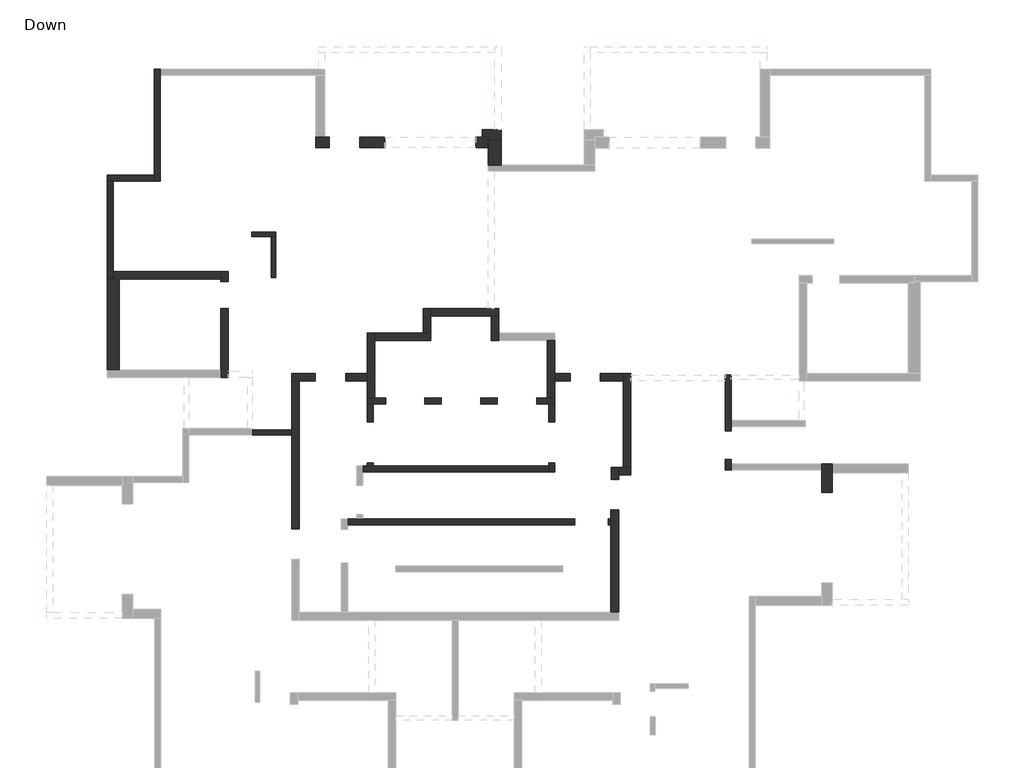
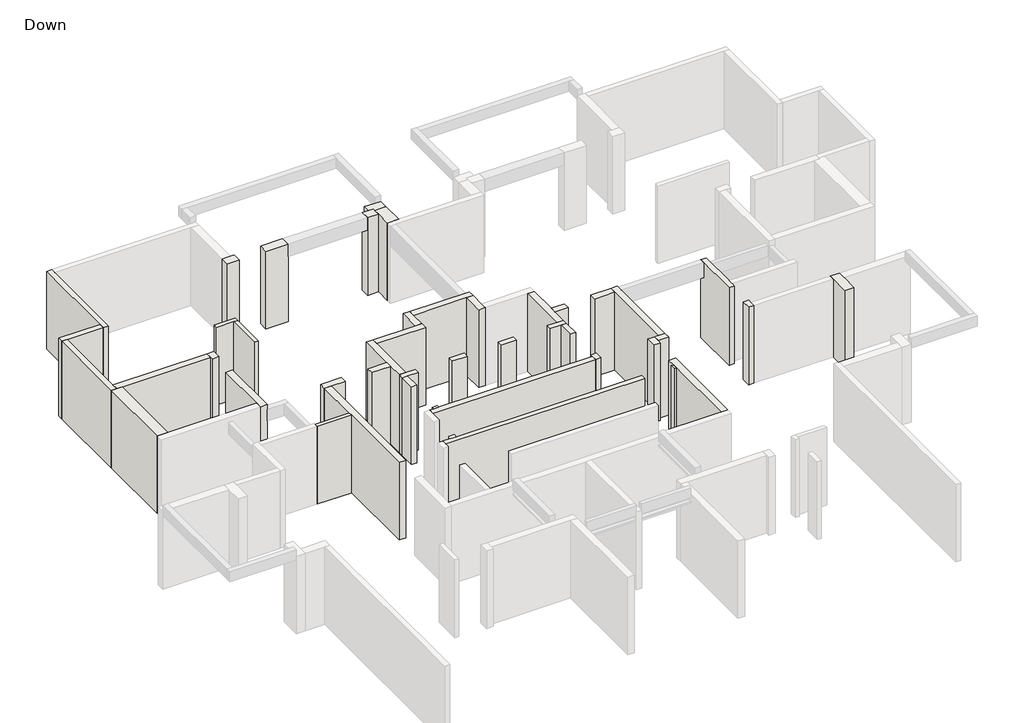
# One storey, part 2 of 3: 44 walls.
"""IFC4 building model written with IfcOpenShell, lengths in millimetres."""

from ifc_helpers import new_model, si_unit, origin, place, context, project, spatial, faceted_brep, element, save

model = new_model("IFC4")

# Units and contexts
model_context = context("Model", 3, world=origin())
ifc_project = project(units=[si_unit("LENGTHUNIT", "METRE", prefix="MILLI")], contexts=[model_context])

# Site, building, storey
site = spatial("IfcSite", under=ifc_project)
building = spatial("IfcBuilding", under=site)
storey = spatial("IfcBuildingStorey", under=building, Name="Down", Elevation=0.0)

# Walls
placement = place(None, origin())
element("IfcWall", 1, ObjectType="15", at=placement, inside=storey, context=model_context, shape_type="Brep", body=[
    faceted_brep([(7954.0579731, -10774.5447275, 0.0), (9252.6267863, -10774.5447275, 0.0), (9252.6267863, -10774.5447275, 2730.0), (9252.6267863, -10774.5447275, 2950.0), (9252.6267863, -10774.5447275, 3100.0), (7954.0579731, -10774.5447275, 3100.0), (7954.0579731, -10624.5447275, 0.0), (7954.0579731, -10624.5447275, 3100.0), (9252.6267863, -10624.5447275, 3100.0), (9252.6267863, -10624.5447275, 0.0)], [[[0, 1, 2, 3, 4, 5]], [[6, 7, 8, 9]], [[1, 0, 6, 9]], [[5, 4, 8, 7]], [[0, 5, 7, 6]], [[4, 3, 2, 1, 9, 8]]]),
])
element("IfcWall", 2, ObjectType="15", at=placement, inside=storey, context=model_context, shape_type="Brep", body=[
    faceted_brep([(7932.894282, -4226.5861029, 0.0), (8577.767247, -4226.5861029, 0.0), (8727.767247, -4226.5861029, 0.0), (8727.767247, -4226.5861029, 3100.0), (8577.767247, -4226.5861029, 3100.0), (7932.894282, -4226.5861029, 3100.0), (7932.894282, -4226.5861029, 2950.0), (7932.894282, -4226.5861029, 2730.0), (7932.894282, -4076.5861029, 0.0), (7932.894282, -4076.5861029, 2730.0), (7932.894282, -4076.5861029, 2950.0), (7932.894282, -4076.5861029, 3100.0), (8727.767247, -4076.5861029, 3100.0), (8727.767247, -4076.5861029, 2950.0), (8727.767247, -4076.5861029, 2730.0), (8727.767247, -4076.5861029, 0.0)], [[[0, 1, 2, 3, 4, 5, 6, 7]], [[8, 9, 10, 11, 12, 13, 14, 15]], [[2, 1, 0, 8, 15]], [[5, 4, 3, 12, 11]], [[0, 7, 6, 5, 11, 10, 9, 8]], [[3, 2, 15, 14, 13, 12]]]),
])
element("IfcWall", 3, ObjectType="15", at=placement, inside=storey, context=model_context, shape_type="Brep", body=[
    faceted_brep([(8577.767247, -4226.5861029, 0.0), (8577.767247, -5575.151797, 0.0), (8577.767247, -5575.151797, 2730.0), (8577.767247, -5575.151797, 2950.0), (8577.767247, -5575.151797, 3100.0), (8577.767247, -4226.5861029, 3100.0), (8577.767247, -4226.5861029, 2950.0), (8577.767247, -4226.5861029, 2730.0), (8727.767247, -4226.5861029, 0.0), (8727.767247, -4226.5861029, 3100.0), (8727.767247, -5575.151797, 3100.0), (8727.767247, -5575.151797, 2950.0), (8727.767247, -5575.151797, 2730.0), (8727.767247, -5575.151797, 0.0)], [[[0, 1, 2, 3, 4, 5, 6, 7]], [[8, 9, 10, 11, 12, 13]], [[1, 0, 8, 13]], [[4, 3, 2, 1, 13, 12, 11, 10]], [[5, 4, 10, 9]], [[0, 7, 6, 5, 9, 8]]]),
])
element("IfcWall", 4, ObjectType="20", at=placement, inside=storey, context=model_context, shape_type="Brep", body=[
    faceted_brep([(4715.8368705, 1316.275118, 0.0), (4715.8368705, -2183.1380866, 0.0), (4715.8368705, -2383.1380866, 0.0), (4715.8368705, -2383.1380866, 3100.0), (4715.8368705, -2183.1380866, 3100.0), (4715.8368705, 1316.275118, 3100.0), (4915.8368705, 1316.275118, 0.0), (4915.8368705, 1316.275118, 3100.0), (4915.8368705, 1116.275118, 3100.0), (4915.8368705, -2383.1380866, 3100.0), (4915.8368705, -2383.1380866, 2950.0), (4915.8368705, -2383.1380866, 2730.0), (4915.8368705, -2383.1380866, 0.0), (4915.8368705, 1116.275118, 0.0)], [[[0, 1, 2, 3, 4, 5]], [[6, 7, 8, 9, 10, 11, 12, 13]], [[2, 1, 0, 6, 13, 12]], [[5, 4, 3, 9, 8, 7]], [[3, 2, 12, 11, 10, 9]], [[0, 5, 7, 6]]]),
])
element("IfcWall", 5, ObjectType="20", at=placement, inside=storey, context=model_context, shape_type="Brep", body=[
    faceted_brep([(4715.8368705, -2183.1380866, 0.0), (3157.3073849, -2183.1380866, 0.0), (3157.3073849, -2183.1380866, 3100.0), (4715.8368705, -2183.1380866, 3100.0), (4715.8368705, -2383.1380866, 0.0), (4715.8368705, -2383.1380866, 3100.0), (3357.3073849, -2383.1380866, 3100.0), (3157.3073849, -2383.1380866, 3100.0), (3157.3073849, -2383.1380866, 0.0), (3357.3073849, -2383.1380866, 0.0)], [[[0, 1, 2, 3]], [[4, 5, 6, 7, 8, 9]], [[1, 0, 4, 9, 8]], [[3, 2, 7, 6, 5]], [[0, 3, 5, 4]], [[2, 1, 8, 7]]]),
])
element("IfcWall", 6, ObjectType="20", at=placement, inside=storey, context=model_context, shape_type="Brep", body=[
    faceted_brep([(3157.3073849, -2383.1380866, 0.0), (3157.3073849, -5626.3894647, 0.0), (3157.3073849, -5626.3894647, 3100.0), (3157.3073849, -2383.1380866, 3100.0), (3357.3073849, -2383.1380866, 0.0), (3357.3073849, -2383.1380866, 2730.0), (3357.3073849, -2383.1380866, 2950.0), (3357.3073849, -2383.1380866, 3100.0), (3357.3073849, -5376.3894647, 3100.0), (3357.3073849, -5626.3894647, 3100.0), (3357.3073849, -5626.3894647, 0.0), (3357.3073849, -5376.3894647, 0.0)], [[[0, 1, 2, 3]], [[4, 5, 6, 7, 8, 9, 10, 11]], [[1, 0, 4, 11, 10]], [[3, 2, 9, 8, 7]], [[0, 3, 7, 6, 5, 4]], [[2, 1, 10, 9]]]),
])
element("IfcWall", 7, ObjectType="20", at=placement, inside=storey, context=model_context, shape_type="Brep", body=[
    faceted_brep([(23780.6220263, -11933.0804512, 0.0), (23780.6220263, -11733.0804512, 0.0), (23780.6220263, -11585.6400699, 0.0), (23780.6220263, -11585.6400699, 3100.0), (23780.6220263, -11733.0804512, 3100.0), (23780.6220263, -11933.0804512, 3100.0), (23580.6220263, -11933.0804512, 0.0), (23580.6220263, -11933.0804512, 2730.0), (23580.6220263, -11933.0804512, 2950.0), (23580.6220263, -11933.0804512, 3100.0), (23580.6220263, -11585.6400699, 3100.0), (23580.6220263, -11585.6400699, 0.0)], [[[0, 1, 2, 3, 4, 5]], [[6, 7, 8, 9, 10, 11]], [[2, 1, 0, 6, 11]], [[3, 2, 11, 10]], [[5, 4, 3, 10, 9]], [[0, 5, 9, 8, 7, 6]]]),
])
element("IfcWall", 8, ObjectType="20", at=placement, inside=storey, context=model_context, shape_type="Brep", body=[
    faceted_brep([(23780.6220263, -10650.7340155, 0.0), (23780.6220263, -10505.7627314, 0.0), (23780.6220263, -10305.7627314, 0.0), (23780.6220263, -8804.7310591, 0.0), (23780.6220263, -8804.7310591, 2300.0), (23780.6220263, -8804.7310591, 2450.0), (23780.6220263, -8804.7310591, 2900.0), (23780.6220263, -8804.7310591, 3100.0), (23780.6220263, -10305.7627314, 3100.0), (23780.6220263, -10505.7627314, 3100.0), (23780.6220263, -10650.7340155, 3100.0), (23580.6220263, -10650.7340155, 0.0), (23580.6220263, -10650.7340155, 3100.0), (23580.6220263, -8804.7310591, 3100.0), (23580.6220263, -8804.7310591, 0.0)], [[[0, 1, 2, 3, 4, 5, 6, 7, 8, 9, 10]], [[11, 12, 13, 14]], [[3, 2, 1, 0, 11, 14]], [[7, 6, 5, 4, 3, 14, 13]], [[10, 9, 8, 7, 13, 12]], [[0, 10, 12, 11]]]),
])
element("IfcWall", 9, ObjectType="20", at=placement, inside=storey, context=model_context, shape_type="Brep", body=[
    faceted_brep([(17955.1365674, -9553.3935127, 0.0), (17705.1365674, -9553.3935127, 0.0), (17354.0877401, -9553.3935127, 0.0), (17354.0877401, -9553.3935127, 3100.0), (17705.1365674, -9553.3935127, 3100.0), (17955.1365674, -9553.3935127, 3100.0), (17955.1365674, -9753.3935127, 0.0), (17955.1365674, -9753.3935127, 3100.0), (17755.1365674, -9753.3935127, 3100.0), (17354.0877401, -9753.3935127, 3100.0), (17354.0877401, -9753.3935127, 2950.0), (17354.0877401, -9753.3935127, 2730.0), (17354.0877401, -9753.3935127, 0.0), (17755.1365674, -9753.3935127, 0.0)], [[[0, 1, 2, 3, 4, 5]], [[6, 7, 8, 9, 10, 11, 12, 13]], [[2, 1, 0, 6, 13, 12]], [[3, 2, 12, 11, 10, 9]], [[5, 4, 3, 9, 8, 7]], [[0, 5, 7, 6]]]),
])
element("IfcWall", 10, ObjectType="20", at=placement, inside=storey, context=model_context, shape_type="Brep", body=[
    faceted_brep([(16055.5189269, -9553.3966318, 0.0), (15504.3811378, -9553.3966318, 0.0), (15504.3811378, -9553.3966318, 2730.0), (15504.3811378, -9553.3966318, 2950.0), (15504.3811378, -9553.3966318, 3100.0), (16055.5189269, -9553.3966318, 3100.0), (16055.5189269, -9553.3966318, 2950.0), (16055.5189269, -9553.3966318, 2730.0), (16055.5189269, -9753.3966318, 0.0), (16055.5189269, -9753.3966318, 2730.0), (16055.5189269, -9753.3966318, 2950.0), (16055.5189269, -9753.3966318, 3100.0), (15504.3811378, -9753.3966318, 3100.0), (15504.3811378, -9753.3966318, 2950.0), (15504.3811378, -9753.3966318, 2730.0), (15504.3811378, -9753.3966318, 0.0)], [[[0, 1, 2, 3, 4, 5, 6, 7]], [[8, 9, 10, 11, 12, 13, 14, 15]], [[1, 0, 8, 15]], [[4, 3, 2, 1, 15, 14, 13, 12]], [[5, 4, 12, 11]], [[0, 7, 6, 5, 11, 10, 9, 8]]]),
])
element("IfcWall", 11, ObjectType="20", at=placement, inside=storey, context=model_context, shape_type="Brep", body=[
    faceted_brep([(14205.8123246, -9553.3966318, 0.0), (13654.4981714, -9553.3966318, 0.0), (13654.4981714, -9553.3966318, 2730.0), (13654.4981714, -9553.3966318, 2950.0), (13654.4981714, -9553.3966318, 3100.0), (14205.8123246, -9553.3966318, 3100.0), (14205.8123246, -9553.3966318, 2950.0), (14205.8123246, -9553.3966318, 2730.0), (14205.8123246, -9753.3966318, 0.0), (14205.8123246, -9753.3966318, 2730.0), (14205.8123246, -9753.3966318, 2950.0), (14205.8123246, -9753.3966318, 3100.0), (13654.4981714, -9753.3966318, 3100.0), (13654.4981714, -9753.3966318, 2950.0), (13654.4981714, -9753.3966318, 2730.0), (13654.4981714, -9753.3966318, 0.0)], [[[0, 1, 2, 3, 4, 5, 6, 7]], [[8, 9, 10, 11, 12, 13, 14, 15]], [[1, 0, 8, 15]], [[4, 3, 2, 1, 15, 14, 13, 12]], [[5, 4, 12, 11]], [[0, 7, 6, 5, 11, 10, 9, 8]]]),
])
element("IfcWall", 12, ObjectType="20", at=placement, inside=storey, context=model_context, shape_type="Brep", body=[
    faceted_brep([(12355.9293582, -9553.3966318, 0.0), (12004.8805309, -9553.3966318, 0.0), (11754.8805309, -9553.3966318, 0.0), (11754.8805309, -9553.3966318, 3100.0), (12004.8805309, -9553.3966318, 3100.0), (12355.9293582, -9553.3966318, 3100.0), (12355.9293582, -9553.3966318, 2950.0), (12355.9293582, -9553.3966318, 2730.0), (12355.9293582, -9753.3966318, 0.0), (12355.9293582, -9753.3966318, 2730.0), (12355.9293582, -9753.3966318, 2950.0), (12355.9293582, -9753.3966318, 3100.0), (11954.8805309, -9753.3966318, 3100.0), (11754.8805309, -9753.3966318, 3100.0), (11754.8805309, -9753.3966318, 0.0), (11954.8805309, -9753.3966318, 0.0)], [[[0, 1, 2, 3, 4, 5, 6, 7]], [[8, 9, 10, 11, 12, 13, 14, 15]], [[2, 1, 0, 8, 15, 14]], [[5, 4, 3, 13, 12, 11]], [[0, 7, 6, 5, 11, 10, 9, 8]], [[3, 2, 14, 13]]]),
])
element("IfcWall", 13, ObjectType="20", at=placement, inside=storey, context=model_context, shape_type="Brep", body=[
    faceted_brep([(11754.8805309, -9753.3966318, 0.0), (11754.8805309, -10353.2077914, 0.0), (11754.8805309, -10353.2077914, 2730.0), (11754.8805309, -10353.2077914, 2950.0), (11754.8805309, -10353.2077914, 3100.0), (11754.8805309, -9753.3966318, 3100.0), (11954.8805309, -9753.3966318, 0.0), (11954.8805309, -9753.3966318, 2730.0), (11954.8805309, -9753.3966318, 2950.0), (11954.8805309, -9753.3966318, 3100.0), (11954.8805309, -10353.2077914, 3100.0), (11954.8805309, -10353.2077914, 2950.0), (11954.8805309, -10353.2077914, 2730.0), (11954.8805309, -10353.2077914, 0.0)], [[[0, 1, 2, 3, 4, 5]], [[6, 7, 8, 9, 10, 11, 12, 13]], [[1, 0, 6, 13]], [[4, 3, 2, 1, 13, 12, 11, 10]], [[5, 4, 10, 9]], [[0, 5, 9, 8, 7, 6]]]),
])
element("IfcWall", 14, ObjectType="20", at=placement, inside=storey, context=model_context, shape_type="Brep", body=[
    faceted_brep([(11754.8805309, -11704.3331041, 0.0), (11754.8805309, -11804.3284255, 0.0), (11754.8805309, -11804.3284255, 2730.0), (11754.8805309, -11804.3284255, 2950.0), (11754.8805309, -11804.3284255, 3100.0), (11754.8805309, -11704.3331041, 3100.0), (11754.8805309, -11704.3331041, 2950.0), (11754.8805309, -11704.3331041, 2730.0), (11954.8805309, -11704.3331041, 0.0), (11954.8805309, -11704.3331041, 2730.0), (11954.8805309, -11704.3331041, 2950.0), (11954.8805309, -11704.3331041, 3100.0), (11954.8805309, -11804.3284255, 3100.0), (11954.8805309, -11804.3284255, 2950.0), (11954.8805309, -11804.3284255, 2730.0), (11954.8805309, -11804.3284255, 0.0)], [[[0, 1, 2, 3, 4, 5, 6, 7]], [[8, 9, 10, 11, 12, 13, 14, 15]], [[1, 0, 8, 15]], [[5, 4, 12, 11]], [[0, 7, 6, 5, 11, 10, 9, 8]], [[4, 3, 2, 1, 15, 14, 13, 12]]]),
])
element("IfcWall", 15, ObjectType="20", at=placement, inside=storey, context=model_context, shape_type="Brep", body=[
    faceted_brep([(11603.5632586, -12004.3284255, 0.0), (17755.1365674, -12004.3284255, 0.0), (17755.1365674, -12004.3284255, 3100.0), (11603.5632586, -12004.3284255, 3100.0), (11603.5632586, -12004.3284255, 2950.0), (11603.5632586, -12004.3284255, 2730.0), (11603.5632586, -11804.3284255, 0.0), (11603.5632586, -11804.3284255, 3100.0), (11754.8805309, -11804.3284255, 3100.0), (11954.8805309, -11804.3284255, 3100.0), (17755.1365674, -11804.3284255, 3100.0), (17755.1365674, -11804.3284255, 2950.0), (17755.1365674, -11804.3284255, 2730.0), (17755.1365674, -11804.3284255, 0.0), (11954.8805309, -11804.3284255, 0.0), (11754.8805309, -11804.3284255, 0.0)], [[[0, 1, 2, 3, 4, 5]], [[6, 7, 8, 9, 10, 11, 12, 13, 14, 15]], [[1, 0, 6, 15, 14, 13]], [[3, 2, 10, 9, 8, 7]], [[2, 1, 13, 12, 11, 10]], [[0, 5, 4, 3, 7, 6]]]),
])
element("IfcWall", 16, ObjectType="20", at=placement, inside=storey, context=model_context, shape_type="Brep", body=[
    faceted_brep([(17955.1365674, -12004.3284255, 0.0), (17955.1365674, -11704.3331041, 0.0), (17955.1365674, -11704.3331041, 2730.0), (17955.1365674, -11704.3331041, 2950.0), (17955.1365674, -11704.3331041, 3100.0), (17955.1365674, -12004.3284255, 3100.0), (17955.1365674, -12004.3284255, 2950.0), (17955.1365674, -12004.3284255, 2730.0), (17755.1365674, -12004.3284255, 0.0), (17755.1365674, -12004.3284255, 3100.0), (17755.1365674, -11804.3284255, 3100.0), (17755.1365674, -11704.3331041, 3100.0), (17755.1365674, -11704.3331041, 2950.0), (17755.1365674, -11704.3331041, 2730.0), (17755.1365674, -11704.3331041, 0.0), (17755.1365674, -11804.3284255, 0.0)], [[[0, 1, 2, 3, 4, 5, 6, 7]], [[8, 9, 10, 11, 12, 13, 14, 15]], [[1, 0, 8, 15, 14]], [[4, 3, 2, 1, 14, 13, 12, 11]], [[5, 4, 11, 10, 9]], [[0, 7, 6, 5, 9, 8]]]),
])
element("IfcWall", 17, ObjectType="20", at=placement, inside=storey, context=model_context, shape_type="Brep", body=[
    faceted_brep([(17755.1365674, -9753.3935127, 0.0), (17755.1365674, -10353.2077914, 0.0), (17755.1365674, -10353.2077914, 2730.0), (17755.1365674, -10353.2077914, 2950.0), (17755.1365674, -10353.2077914, 3100.0), (17755.1365674, -9753.3935127, 3100.0), (17755.1365674, -9753.3935127, 2950.0), (17755.1365674, -9753.3935127, 2730.0), (17955.1365674, -9753.3935127, 0.0), (17955.1365674, -9753.3935127, 3100.0), (17955.1365674, -10353.2077914, 3100.0), (17955.1365674, -10353.2077914, 2950.0), (17955.1365674, -10353.2077914, 2730.0), (17955.1365674, -10353.2077914, 0.0)], [[[0, 1, 2, 3, 4, 5, 6, 7]], [[8, 9, 10, 11, 12, 13]], [[1, 0, 8, 13]], [[4, 3, 2, 1, 13, 12, 11, 10]], [[5, 4, 10, 9]], [[0, 7, 6, 5, 9, 8]]]),
])
element("IfcWall", 18, ObjectType="20", at=placement, inside=storey, context=model_context, shape_type="Brep", body=[
    faceted_brep([(11100.0437745, -13752.8020387, 0.0), (18611.3873556, -13752.8020387, 0.0), (18611.3873556, -13752.8020387, 2730.0), (18611.3873556, -13752.8020387, 2950.0), (18611.3873556, -13752.8020387, 3100.0), (11100.0437745, -13752.8020387, 3100.0), (11100.0437745, -13752.8020387, 2950.0), (11100.0437745, -13752.8020387, 2730.0), (11100.0437745, -13552.8020387, 0.0), (11100.0437745, -13552.8020387, 3100.0), (11403.5632586, -13552.8020387, 3100.0), (11603.5632586, -13552.8020387, 3100.0), (18611.3873556, -13552.8020387, 3100.0), (18611.3873556, -13552.8020387, 2950.0), (18611.3873556, -13552.8020387, 2730.0), (18611.3873556, -13552.8020387, 0.0), (11603.5632586, -13552.8020387, 0.0), (11403.5632586, -13552.8020387, 0.0)], [[[0, 1, 2, 3, 4, 5, 6, 7]], [[8, 9, 10, 11, 12, 13, 14, 15, 16, 17]], [[1, 0, 8, 17, 16, 15]], [[4, 3, 2, 1, 15, 14, 13, 12]], [[5, 4, 12, 11, 10, 9]], [[0, 7, 6, 5, 9, 8]]]),
])
element("IfcWall", 19, ObjectType="20", at=placement, inside=storey, context=model_context, shape_type="Brep", body=[
    faceted_brep([(19712.4283852, -13752.8020387, 0.0), (19808.6310988, -13752.8020387, 0.0), (19808.6310988, -13752.8020387, 2730.0), (19808.6310988, -13752.8020387, 2950.0), (19808.6310988, -13752.8020387, 3100.0), (19712.4283852, -13752.8020387, 3100.0), (19712.4283852, -13752.8020387, 2950.0), (19712.4283852, -13752.8020387, 2730.0), (19712.4283852, -13552.8020387, 0.0), (19712.4283852, -13552.8020387, 2730.0), (19712.4283852, -13552.8020387, 2950.0), (19712.4283852, -13552.8020387, 3100.0), (19808.6310988, -13552.8020387, 3100.0), (19808.6310988, -13552.8020387, 2950.0), (19808.6310988, -13552.8020387, 2730.0), (19808.6310988, -13552.8020387, 0.0)], [[[0, 1, 2, 3, 4, 5, 6, 7]], [[8, 9, 10, 11, 12, 13, 14, 15]], [[1, 0, 8, 15]], [[5, 4, 12, 11]], [[0, 7, 6, 5, 11, 10, 9, 8]], [[4, 3, 2, 1, 15, 14, 13, 12]]]),
])
element("IfcWall", 20, ObjectType="25", at=placement, inside=storey, context=model_context, shape_type="Brep", body=[
    faceted_brep([(6907.9504595, -5376.3894647, 0.0), (3357.3073849, -5376.3894647, 0.0), (3357.3073849, -5376.3894647, 2730.0), (3357.3073849, -5376.3894647, 2950.0), (3357.3073849, -5376.3894647, 3100.0), (6907.9504595, -5376.3894647, 3100.0), (6907.9504595, -5626.3894647, 0.0), (6907.9504595, -5626.3894647, 2730.0), (6907.9504595, -5626.3894647, 2950.0), (6907.9504595, -5626.3894647, 3100.0), (3557.3073849, -5626.3894647, 3100.0), (3357.3073849, -5626.3894647, 3100.0), (3357.3073849, -5626.3894647, 0.0), (3557.3073849, -5626.3894647, 0.0)], [[[0, 1, 2, 3, 4, 5]], [[6, 7, 8, 9, 10, 11, 12, 13]], [[1, 0, 6, 13, 12]], [[5, 4, 11, 10, 9]], [[4, 3, 2, 1, 12, 11]], [[0, 5, 9, 8, 7, 6]]]),
])
element("IfcWall", 21, ObjectType="25", at=placement, inside=storey, context=model_context, shape_type="Brep", body=[
    faceted_brep([(6907.9504595, -5376.3894647, 0.0), (6907.9504595, -5626.3894647, 0.0), (6907.9504595, -5710.0703278, 0.0), (6907.9504595, -5710.0703278, 2730.0), (6907.9504595, -5710.0703278, 2950.0), (6907.9504595, -5710.0703278, 3100.0), (6907.9504595, -5626.3894647, 3100.0), (6907.9504595, -5376.3894647, 3100.0), (7157.9504595, -5376.3894647, 0.0), (7157.9504595, -5376.3894647, 2730.0), (7157.9504595, -5376.3894647, 2950.0), (7157.9504595, -5376.3894647, 3100.0), (7157.9504595, -5710.0703278, 3100.0), (7157.9504595, -5710.0703278, 2950.0), (7157.9504595, -5710.0703278, 2730.0), (7157.9504595, -5710.0703278, 0.0)], [[[0, 1, 2, 3, 4, 5, 6, 7]], [[8, 9, 10, 11, 12, 13, 14, 15]], [[2, 1, 0, 8, 15]], [[5, 4, 3, 2, 15, 14, 13, 12]], [[7, 6, 5, 12, 11]], [[0, 7, 11, 10, 9, 8]]]),
])
element("IfcWall", 22, ObjectType="25", at=placement, inside=storey, context=model_context, shape_type="Brep", body=[
    faceted_brep([(6907.9504595, -6598.7689899, 0.0), (6907.9504595, -8625.9821525, 0.0), (6907.9504595, -8875.9821525, 0.0), (6907.9504595, -8875.9821525, 3100.0), (6907.9504595, -8625.9821525, 3100.0), (6907.9504595, -6598.7689899, 3100.0), (6907.9504595, -6598.7689899, 2950.0), (6907.9504595, -6598.7689899, 2730.0), (7157.9504595, -6598.7689899, 0.0), (7157.9504595, -6598.7689899, 2730.0), (7157.9504595, -6598.7689899, 2950.0), (7157.9504595, -6598.7689899, 3100.0), (7157.9504595, -8875.9821525, 3100.0), (7157.9504595, -8875.9821525, 2450.0), (7157.9504595, -8875.9821525, 2300.0), (7157.9504595, -8875.9821525, 0.0)], [[[0, 1, 2, 3, 4, 5, 6, 7]], [[8, 9, 10, 11, 12, 13, 14, 15]], [[2, 1, 0, 8, 15]], [[5, 4, 3, 12, 11]], [[0, 7, 6, 5, 11, 10, 9, 8]], [[3, 2, 15, 14, 13, 12]]]),
])
element("IfcWall", 23, ObjectType="25", at=placement, inside=storey, context=model_context, shape_type="Brep", body=[
    faceted_brep([(10036.3888134, -8753.4091082, 0.0), (9252.6267863, -8753.4091082, 0.0), (9252.6267863, -8753.4091082, 2730.0), (9252.6267863, -8753.4091082, 2950.0), (9252.6267863, -8753.4091082, 3100.0), (10036.3888134, -8753.4091082, 3100.0), (10036.3888134, -8753.4091082, 2950.0), (10036.3888134, -8753.4091082, 2730.0), (10036.3888134, -9003.4091082, 0.0), (10036.3888134, -9003.4091082, 2730.0), (10036.3888134, -9003.4091082, 2950.0), (10036.3888134, -9003.4091082, 3100.0), (9502.6267863, -9003.4091082, 3100.0), (9252.6267863, -9003.4091082, 3100.0), (9252.6267863, -9003.4091082, 0.0), (9502.6267863, -9003.4091082, 0.0)], [[[0, 1, 2, 3, 4, 5, 6, 7]], [[8, 9, 10, 11, 12, 13, 14, 15]], [[1, 0, 8, 15, 14]], [[5, 4, 13, 12, 11]], [[0, 7, 6, 5, 11, 10, 9, 8]], [[4, 3, 2, 1, 14, 13]]]),
])
element("IfcWall", 24, ObjectType="25", at=placement, inside=storey, context=model_context, shape_type="Brep", body=[
    faceted_brep([(9252.6267863, -9003.4091082, 0.0), (9252.6267863, -10624.5447275, 0.0), (9252.6267863, -10774.5447275, 0.0), (9252.6267863, -13892.8351282, 0.0), (9252.6267863, -13892.8351282, 3100.0), (9252.6267863, -10774.5447275, 3100.0), (9252.6267863, -10624.5447275, 3100.0), (9252.6267863, -9003.4091082, 3100.0), (9502.6267863, -9003.4091082, 0.0), (9502.6267863, -9003.4091082, 2730.0), (9502.6267863, -9003.4091082, 2950.0), (9502.6267863, -9003.4091082, 3100.0), (9502.6267863, -13892.8351282, 3100.0), (9502.6267863, -13892.8351282, 0.0)], [[[0, 1, 2, 3, 4, 5, 6, 7]], [[8, 9, 10, 11, 12, 13]], [[3, 2, 1, 0, 8, 13]], [[4, 3, 13, 12]], [[7, 6, 5, 4, 12, 11]], [[0, 7, 11, 10, 9, 8]]]),
])
element("IfcWall", 25, ObjectType="25", at=placement, inside=storey, context=model_context, shape_type="Brep", body=[
    faceted_brep([(20058.6310988, -16656.0156488, 0.0), (20058.6310988, -13252.8098364, 0.0), (20058.6310988, -13252.8098364, 3100.0), (20058.6310988, -16656.0156488, 3100.0), (19808.6310988, -16656.0156488, 0.0), (19808.6310988, -16656.0156488, 3100.0), (19808.6310988, -13752.8020387, 3100.0), (19808.6310988, -13552.8020387, 3100.0), (19808.6310988, -13252.8098364, 3100.0), (19808.6310988, -13252.8098364, 0.0), (19808.6310988, -13552.8020387, 0.0), (19808.6310988, -13752.8020387, 0.0)], [[[0, 1, 2, 3]], [[4, 5, 6, 7, 8, 9, 10, 11]], [[1, 0, 4, 11, 10, 9]], [[2, 1, 9, 8]], [[3, 2, 8, 7, 6, 5]], [[0, 3, 5, 4]]]),
])
element("IfcWall", 26, ObjectType="25", at=placement, inside=storey, context=model_context, shape_type="Brep", body=[
    faceted_brep([(20059.9577283, -12254.2363446, 0.0), (20059.9577283, -12106.7116801, 0.0), (20059.9577283, -11856.7116801, 0.0), (20059.9577283, -11856.7116801, 3100.0), (20059.9577283, -12106.7116801, 3100.0), (20059.9577283, -12254.2363446, 3100.0), (19809.9577283, -12254.2363446, 0.0), (19809.9577283, -12254.2363446, 3100.0), (19809.9577283, -11856.7116801, 3100.0), (19809.9577283, -11856.7116801, 0.0)], [[[0, 1, 2, 3, 4, 5]], [[6, 7, 8, 9]], [[2, 1, 0, 6, 9]], [[5, 4, 3, 8, 7]], [[0, 5, 7, 6]], [[3, 2, 9, 8]]]),
])
element("IfcWall", 27, ObjectType="25", at=placement, inside=storey, context=model_context, shape_type="Brep", body=[
    faceted_brep([(20059.9577283, -12106.7116801, 0.0), (20461.0939579, -12106.7116801, 0.0), (20461.0939579, -12106.7116801, 2730.0), (20461.0939579, -12106.7116801, 2950.0), (20461.0939579, -12106.7116801, 3100.0), (20059.9577283, -12106.7116801, 3100.0), (20059.9577283, -12106.7116801, 2950.0), (20059.9577283, -12106.7116801, 2730.0), (20059.9577283, -11856.7116801, 0.0), (20059.9577283, -11856.7116801, 3100.0), (20211.0939579, -11856.7116801, 3100.0), (20461.0939579, -11856.7116801, 3100.0), (20461.0939579, -11856.7116801, 0.0), (20211.0939579, -11856.7116801, 0.0)], [[[0, 1, 2, 3, 4, 5, 6, 7]], [[8, 9, 10, 11, 12, 13]], [[1, 0, 8, 13, 12]], [[5, 4, 11, 10, 9]], [[0, 7, 6, 5, 9, 8]], [[4, 3, 2, 1, 12, 11]]]),
])
element("IfcWall", 28, ObjectType="25", at=placement, inside=storey, context=model_context, shape_type="Brep", body=[
    faceted_brep([(20461.0939579, -11856.7116801, 0.0), (20461.0939579, -8753.4091082, 0.0), (20461.0939579, -8753.4091082, 2730.0), (20461.0939579, -8753.4091082, 2950.0), (20461.0939579, -8753.4091082, 3100.0), (20461.0939579, -11856.7116801, 3100.0), (20211.0939579, -11856.7116801, 0.0), (20211.0939579, -11856.7116801, 2730.0), (20211.0939579, -11856.7116801, 2950.0), (20211.0939579, -11856.7116801, 3100.0), (20211.0939579, -9003.4091082, 3100.0), (20211.0939579, -8753.4091082, 3100.0), (20211.0939579, -8753.4091082, 0.0), (20211.0939579, -9003.4091082, 0.0)], [[[0, 1, 2, 3, 4, 5]], [[6, 7, 8, 9, 10, 11, 12, 13]], [[1, 0, 6, 13, 12]], [[5, 4, 11, 10, 9]], [[0, 5, 9, 8, 7, 6]], [[4, 3, 2, 1, 12, 11]]]),
])
element("IfcWall", 29, ObjectType="25", at=placement, inside=storey, context=model_context, shape_type="Brep", body=[
    faceted_brep([(20211.0939579, -8753.4091082, 0.0), (19458.8168201, -8753.4091082, 0.0), (19458.8168201, -8753.4091082, 3100.0), (20211.0939579, -8753.4091082, 3100.0), (20211.0939579, -9003.4091082, 0.0), (20211.0939579, -9003.4091082, 2730.0), (20211.0939579, -9003.4091082, 2950.0), (20211.0939579, -9003.4091082, 3100.0), (19458.8168201, -9003.4091082, 3100.0), (19458.8168201, -9003.4091082, 0.0)], [[[0, 1, 2, 3]], [[4, 5, 6, 7, 8, 9]], [[1, 0, 4, 9]], [[2, 1, 9, 8]], [[3, 2, 8, 7]], [[0, 3, 7, 6, 5, 4]]]),
])
element("IfcWall", 30, ObjectType="25", at=placement, inside=storey, context=model_context, shape_type="Brep", body=[
    faceted_brep([(18458.8324156, -8753.4091082, 0.0), (17955.1365674, -8753.4091082, 0.0), (17955.1365674, -8753.4091082, 2730.0), (17955.1365674, -8753.4091082, 2950.0), (17955.1365674, -8753.4091082, 3100.0), (18458.8324156, -8753.4091082, 3100.0), (18458.8324156, -9003.4091082, 0.0), (18458.8324156, -9003.4091082, 3100.0), (17955.1365674, -9003.4091082, 3100.0), (17955.1365674, -9003.4091082, 2950.0), (17955.1365674, -9003.4091082, 2730.0), (17955.1365674, -9003.4091082, 0.0)], [[[0, 1, 2, 3, 4, 5]], [[6, 7, 8, 9, 10, 11]], [[1, 0, 6, 11]], [[5, 4, 8, 7]], [[0, 5, 7, 6]], [[4, 3, 2, 1, 11, 10, 9, 8]]]),
])
element("IfcWall", 31, ObjectType="25", at=placement, inside=storey, context=model_context, shape_type="Brep", body=[
    faceted_brep([(11034.9623053, -9003.4091082, 0.0), (11754.8805309, -9003.4091082, 0.0), (11754.8805309, -9003.4091082, 2730.0), (11754.8805309, -9003.4091082, 2950.0), (11754.8805309, -9003.4091082, 3100.0), (11034.9623053, -9003.4091082, 3100.0), (11034.9623053, -9003.4091082, 2950.0), (11034.9623053, -9003.4091082, 2730.0), (11034.9623053, -8753.4091082, 0.0), (11034.9623053, -8753.4091082, 2730.0), (11034.9623053, -8753.4091082, 2950.0), (11034.9623053, -8753.4091082, 3100.0), (11754.8805309, -8753.4091082, 3100.0), (11754.8805309, -8753.4091082, 2950.0), (11754.8805309, -8753.4091082, 2730.0), (11754.8805309, -8753.4091082, 0.0)], [[[0, 1, 2, 3, 4, 5, 6, 7]], [[8, 9, 10, 11, 12, 13, 14, 15]], [[1, 0, 8, 15]], [[5, 4, 12, 11]], [[0, 7, 6, 5, 11, 10, 9, 8]], [[4, 3, 2, 1, 15, 14, 13, 12]]]),
])
element("IfcWall", 32, ObjectType="25", at=placement, inside=storey, context=model_context, shape_type="Brep", body=[
    faceted_brep([(12004.8805309, -9553.3966318, 0.0), (12004.8805309, -7653.6947082, 0.0), (12004.8805309, -7403.6947082, 0.0), (12004.8805309, -7403.6947082, 3100.0), (12004.8805309, -7653.6947082, 3100.0), (12004.8805309, -9553.3966318, 3100.0), (11754.8805309, -9553.3966318, 0.0), (11754.8805309, -9553.3966318, 3100.0), (11754.8805309, -9003.4091082, 3100.0), (11754.8805309, -8753.4091082, 3100.0), (11754.8805309, -7403.6947082, 3100.0), (11754.8805309, -7403.6947082, 2950.0), (11754.8805309, -7403.6947082, 2730.0), (11754.8805309, -7403.6947082, 0.0), (11754.8805309, -8753.4091082, 0.0), (11754.8805309, -9003.4091082, 0.0)], [[[0, 1, 2, 3, 4, 5]], [[6, 7, 8, 9, 10, 11, 12, 13, 14, 15]], [[2, 1, 0, 6, 15, 14, 13]], [[5, 4, 3, 10, 9, 8, 7]], [[3, 2, 13, 12, 11, 10]], [[0, 5, 7, 6]]]),
])
element("IfcWall", 33, ObjectType="25", at=placement, inside=storey, context=model_context, shape_type="Brep", body=[
    faceted_brep([(12004.8805309, -7653.6947082, 0.0), (13854.4950523, -7653.6947082, 0.0), (13854.4950523, -7653.6947082, 3100.0), (12004.8805309, -7653.6947082, 3100.0), (12004.8805309, -7403.6947082, 0.0), (12004.8805309, -7403.6947082, 3100.0), (13604.4950523, -7403.6947082, 3100.0), (13854.4950523, -7403.6947082, 3100.0), (13854.4950523, -7403.6947082, 0.0), (13604.4950523, -7403.6947082, 0.0)], [[[0, 1, 2, 3]], [[4, 5, 6, 7, 8, 9]], [[1, 0, 4, 9, 8]], [[3, 2, 7, 6, 5]], [[0, 3, 5, 4]], [[2, 1, 8, 7]]]),
])
element("IfcWall", 34, ObjectType="25", at=placement, inside=storey, context=model_context, shape_type="Brep", body=[
    faceted_brep([(13854.4950523, -7403.6947082, 0.0), (13854.4950523, -6853.7071845, 0.0), (13854.4950523, -6603.7071845, 0.0), (13854.4950523, -6603.7071845, 3100.0), (13854.4950523, -6853.7071845, 3100.0), (13854.4950523, -7403.6947082, 3100.0), (13604.4950523, -7403.6947082, 0.0), (13604.4950523, -7403.6947082, 2730.0), (13604.4950523, -7403.6947082, 2950.0), (13604.4950523, -7403.6947082, 3100.0), (13604.4950523, -6603.7071845, 3100.0), (13604.4950523, -6603.7071845, 2950.0), (13604.4950523, -6603.7071845, 2730.0), (13604.4950523, -6603.7071845, 0.0)], [[[0, 1, 2, 3, 4, 5]], [[6, 7, 8, 9, 10, 11, 12, 13]], [[2, 1, 0, 6, 13]], [[5, 4, 3, 10, 9]], [[0, 5, 9, 8, 7, 6]], [[3, 2, 13, 12, 11, 10]]]),
])
element("IfcWall", 35, ObjectType="25", at=placement, inside=storey, context=model_context, shape_type="Brep", body=[
    faceted_brep([(13854.4950523, -6853.7071845, 0.0), (15855.4299651, -6853.7071845, 0.0), (16105.4299651, -6853.7071845, 0.0), (16105.4299651, -6853.7071845, 3100.0), (15855.4299651, -6853.7071845, 3100.0), (13854.4950523, -6853.7071845, 3100.0), (13854.4950523, -6603.7071845, 0.0), (13854.4950523, -6603.7071845, 3100.0), (16105.4299651, -6603.7071845, 3100.0), (16105.4299651, -6603.7071845, 2950.0), (16105.4299651, -6603.7071845, 2730.0), (16105.4299651, -6603.7071845, 0.0)], [[[0, 1, 2, 3, 4, 5]], [[6, 7, 8, 9, 10, 11]], [[2, 1, 0, 6, 11]], [[5, 4, 3, 8, 7]], [[0, 5, 7, 6]], [[3, 2, 11, 10, 9, 8]]]),
])
element("IfcWall", 36, ObjectType="25", at=placement, inside=storey, context=model_context, shape_type="Brep", body=[
    faceted_brep([(15855.4299651, -6853.7071845, 0.0), (15855.4299651, -7653.6026273, 0.0), (15855.4299651, -7653.6026273, 3100.0), (15855.4299651, -6853.7071845, 3100.0), (16105.4299651, -6853.7071845, 0.0), (16105.4299651, -6853.7071845, 3100.0), (16105.4299651, -7403.6026273, 3100.0), (16105.4299651, -7653.6026273, 3100.0), (16105.4299651, -7653.6026273, 0.0), (16105.4299651, -7403.6026273, 0.0)], [[[0, 1, 2, 3]], [[4, 5, 6, 7, 8, 9]], [[1, 0, 4, 9, 8]], [[3, 2, 7, 6, 5]], [[0, 3, 5, 4]], [[2, 1, 8, 7]]]),
])
element("IfcWall", 37, ObjectType="25", at=placement, inside=storey, context=model_context, shape_type="Brep", body=[
    faceted_brep([(17705.1365674, -7653.6026273, 0.0), (17705.1365674, -9553.3935127, 0.0), (17705.1365674, -9553.3935127, 3100.0), (17705.1365674, -7653.6026273, 3100.0), (17955.1365674, -7653.6026273, 0.0), (17955.1365674, -7653.6026273, 3100.0), (17955.1365674, -8753.4091082, 3100.0), (17955.1365674, -9003.4091082, 3100.0), (17955.1365674, -9553.3935127, 3100.0), (17955.1365674, -9553.3935127, 0.0), (17955.1365674, -9003.4091082, 0.0), (17955.1365674, -8753.4091082, 0.0)], [[[0, 1, 2, 3]], [[4, 5, 6, 7, 8, 9, 10, 11]], [[1, 0, 4, 11, 10, 9]], [[3, 2, 8, 7, 6, 5]], [[0, 3, 5, 4]], [[2, 1, 9, 8]]]),
])
element("IfcWall", 38, ObjectType="35", at=placement, inside=storey, context=model_context, shape_type="Brep", body=[
    faceted_brep([(10045.0259753, -1285.8943434, 0.0), (10497.5809154, -1285.8943434, 0.0), (10497.5809154, -1285.8943434, 2730.0), (10497.5809154, -1285.8943434, 2950.0), (10497.5809154, -1285.8943434, 3100.0), (10045.0259753, -1285.8943434, 3100.0), (10045.0259753, -1285.8943434, 2950.0), (10045.0259753, -1285.8943434, 2730.0), (10045.0259753, -935.8943434, 0.0), (10045.0259753, -935.8943434, 3100.0), (10345.0259753, -935.8943434, 3100.0), (10497.5809154, -935.8943434, 3100.0), (10497.5809154, -935.8943434, 2950.0), (10497.5809154, -935.8943434, 2730.0), (10497.5809154, -935.8943434, 0.0), (10345.0259753, -935.8943434, 0.0)], [[[0, 1, 2, 3, 4, 5, 6, 7]], [[8, 9, 10, 11, 12, 13, 14, 15]], [[1, 0, 8, 15, 14]], [[4, 3, 2, 1, 14, 13, 12, 11]], [[5, 4, 11, 10, 9]], [[0, 7, 6, 5, 9, 8]]]),
])
element("IfcWall", 39, ObjectType="35", at=placement, inside=storey, context=model_context, shape_type="Brep", body=[
    faceted_brep([(11496.1544072, -1285.8943434, 0.0), (12338.469313, -1285.8943434, 0.0), (12338.469313, -1285.8943434, 2600.0), (12338.469313, -1285.8943434, 3100.0), (11496.1544072, -1285.8943434, 3100.0), (11496.1544072, -1285.8943434, 2950.0), (11496.1544072, -1285.8943434, 2730.0), (11496.1544072, -935.8943434, 0.0), (11496.1544072, -935.8943434, 2730.0), (11496.1544072, -935.8943434, 2950.0), (11496.1544072, -935.8943434, 3100.0), (12338.469313, -935.8943434, 3100.0), (12338.469313, -935.8943434, 2600.0), (12338.469313, -935.8943434, 0.0)], [[[0, 1, 2, 3, 4, 5, 6]], [[7, 8, 9, 10, 11, 12, 13]], [[1, 0, 7, 13]], [[3, 2, 1, 13, 12, 11]], [[4, 3, 11, 10]], [[0, 6, 5, 4, 10, 9, 8, 7]]]),
])
element("IfcWall", 40, ObjectType="35", at=placement, inside=storey, context=model_context, shape_type="Brep", body=[
    faceted_brep([(27127.656655, -12677.8628948, 0.0), (27127.656655, -12033.0804512, 0.0), (27127.656655, -11733.0804512, 0.0), (27127.656655, -11733.0804512, 3100.0), (27127.656655, -12033.0804512, 3100.0), (27127.656655, -12677.8628948, 3100.0), (27127.656655, -12677.8628948, 2950.0), (27127.656655, -12677.8628948, 2730.0), (26777.656655, -12677.8628948, 0.0), (26777.656655, -12677.8628948, 2730.0), (26777.656655, -12677.8628948, 2950.0), (26777.656655, -12677.8628948, 3100.0), (26777.656655, -11933.0804512, 3100.0), (26777.656655, -11733.0804512, 3100.0), (26777.656655, -11733.0804512, 0.0), (26777.656655, -11933.0804512, 0.0)], [[[0, 1, 2, 3, 4, 5, 6, 7]], [[8, 9, 10, 11, 12, 13, 14, 15]], [[2, 1, 0, 8, 15, 14]], [[5, 4, 3, 13, 12, 11]], [[0, 7, 6, 5, 11, 10, 9, 8]], [[3, 2, 14, 13]]]),
])
element("IfcWall", 41, ObjectType="35", at=placement, inside=storey, context=model_context, shape_type="Brep", body=[
    faceted_brep([(15339.3043472, -1285.8943434, 0.0), (15752.9774125, -1285.8943434, 0.0), (15752.9774125, -1285.8943434, 2730.0), (15752.9774125, -1285.8943434, 2950.0), (15752.9774125, -1285.8943434, 3100.0), (15339.3043472, -1285.8943434, 3100.0), (15339.3043472, -1285.8943434, 2600.0), (15339.3043472, -935.8943434, 0.0), (15339.3043472, -935.8943434, 2600.0), (15339.3043472, -935.8943434, 3100.0), (15559.2303705, -935.8943434, 3100.0), (15752.9774125, -935.8943434, 3100.0), (15752.9774125, -935.8943434, 0.0), (15559.2303705, -935.8943434, 0.0), (15752.9774125, -1035.8100602, 0.0), (15752.9774125, -1035.8100602, 3100.0)], [[[0, 1, 2, 3, 4, 5, 6]], [[7, 8, 9, 10, 11, 12, 13]], [[1, 0, 7, 13, 12, 14]], [[5, 4, 15, 11, 10, 9]], [[0, 6, 5, 9, 8, 7]], [[4, 3, 2, 1, 14, 12, 11, 15]]]),
])
element("IfcWall", 42, ObjectType="35", at=placement, inside=storey, context=model_context, shape_type="Brep", body=[
    faceted_brep([(16172.9774125, -1035.8100602, 0.0), (16172.9774125, -1035.8100602, 3100.0), (15752.9774125, -1035.8100602, 3100.0), (15752.9774125, -1035.8100602, 0.0), (16172.9774125, -685.8100602, 0.0), (15559.2303705, -685.8100602, 0.0), (15559.2303705, -685.8100602, 2730.0), (15559.2303705, -685.8100602, 2950.0), (15559.2303705, -685.8100602, 3100.0), (16172.9774125, -685.8100602, 3100.0), (16172.9774125, -685.8100602, 2950.0), (16172.9774125, -685.8100602, 2730.0), (15752.9774125, -935.8943434, 0.0), (15559.2303705, -935.8943434, 0.0), (15559.2303705, -935.8943434, 3100.0), (15752.9774125, -935.8943434, 3100.0), (15559.2303705, -935.8943434, 2730.0), (15559.2303705, -935.8943434, 2950.0)], [[[0, 1, 2, 3]], [[4, 5, 6, 7, 8, 9, 10, 11]], [[5, 4, 0, 3, 12, 13]], [[9, 8, 14, 15, 2, 1]], [[8, 7, 6, 5, 13, 16, 17, 14]], [[1, 0, 4, 11, 10, 9]], [[12, 15, 14, 17, 16, 13]], [[15, 12, 3, 2]]]),
])
element("IfcWall", 43, ObjectType="40", at=placement, inside=storey, context=model_context, shape_type="Brep", body=[
    faceted_brep([(3557.3073849, -8625.9821525, 0.0), (3557.3073849, -5626.3894647, 0.0), (3557.3073849, -5626.3894647, 2730.0), (3557.3073849, -5626.3894647, 2950.0), (3557.3073849, -5626.3894647, 3100.0), (3557.3073849, -8625.9821525, 3100.0), (3557.3073849, -8625.9821525, 2950.0), (3557.3073849, -8625.9821525, 2730.0), (3157.3073849, -8625.9821525, 0.0), (3157.3073849, -8625.9821525, 3100.0), (3157.3073849, -5626.3894647, 3100.0), (3157.3073849, -5626.3894647, 0.0), (3357.3073849, -5626.3894647, 0.0), (3357.3073849, -5626.3894647, 3100.0)], [[[0, 1, 2, 3, 4, 5, 6, 7]], [[8, 9, 10, 11]], [[1, 0, 8, 11, 12]], [[5, 4, 13, 10, 9]], [[4, 3, 2, 1, 12, 11, 10, 13]], [[0, 7, 6, 5, 9, 8]]]),
])
element("IfcWall", 44, ObjectType="42", at=placement, inside=storey, context=model_context, shape_type="Brep", body=[
    faceted_brep([(15752.9774125, -1035.8100602, 0.0), (15752.9774125, -1285.8943434, 0.0), (15752.9774125, -1861.9790741, 0.0), (15752.9774125, -1861.9790741, 3100.0), (15752.9774125, -1285.8943434, 3100.0), (15752.9774125, -1035.8100602, 3100.0), (16172.9774125, -1035.8100602, 0.0), (16172.9774125, -1035.8100602, 3100.0), (16172.9774125, -1861.9790741, 3100.0), (16172.9774125, -1861.9790741, 0.0)], [[[0, 1, 2, 3, 4, 5]], [[6, 7, 8, 9]], [[2, 1, 0, 6, 9]], [[5, 4, 3, 8, 7]], [[3, 2, 9, 8]], [[0, 5, 7, 6]]]),
])

save(model, "model.ifc")

# Revit data of these elements
# Type "15"
#   Layers, outside or top first: 15 cm "Concrete" (function 1)
# Type "20"
#   Layers, outside or top first: 20 cm "Concrete" (function 1)
# Type "25"
#   Layers, outside or top first: 25 cm "Concrete" (function 1)
# Type "35"
#   Layers, outside or top first: 35 cm "Concrete" (function 1)
# Type "40"
#   Layers, outside or top first: 40 cm "Concrete" (function 1)
# Type "42"
#   Layers, outside or top first: 42 cm "Concrete" (function 1)
# Element 1 (IfcWall, "15")
#   Comments = ""
#   Mark = "W100"
#   SOFiSTiK_EdgeZones = "W104"
#   SOFiSTiK_AMG_Comments = ""
#   Top Offset = 0 cm
#   Base Offset = 0 cm
#   wall height = 310 cm
#   SOFiSTiK_AMG_Scheduled = yes
#   SOFiSTiK_AMG_Adjusted = yes
#   Phase Created = New Construction
#   Base Constraint = Down
#   Top Constraint = Typical Floor
#   Materials on its faces: "Concrete"
# Element 2 (IfcWall, "15")
#   Comments = ""
#   Mark = "W101"
#   SOFiSTiK_EdgeZones = "W105"
#   SOFiSTiK_AMG_Comments = ""
#   Top Offset = 0 cm
#   Base Offset = 0 cm
#   wall height = 310 cm
#   SOFiSTiK_AMG_Scheduled = yes
#   SOFiSTiK_AMG_Adjusted = yes
#   Phase Created = New Construction
#   Base Constraint = Down
#   Top Constraint = Typical Floor
#   Materials on its faces: "Concrete"
# Element 3 (IfcWall, "15")
#   Comments = ""
#   Mark = "W102"
#   SOFiSTiK_EdgeZones = "W106"
#   SOFiSTiK_AMG_Comments = ""
#   Top Offset = 0 cm
#   Base Offset = 0 cm
#   wall height = 310 cm
#   SOFiSTiK_AMG_Scheduled = yes
#   SOFiSTiK_AMG_Adjusted = yes
#   Phase Created = New Construction
#   Base Constraint = Down
#   Top Constraint = Typical Floor
#   Materials on its faces: "Concrete"
# Element 4 (IfcWall, "20")
#   Comments = ""
#   Mark = "W1"
#   SOFiSTiK_EdgeZones = "W1"
#   SOFiSTiK_AMG_Comments = ""
#   Top Offset = 0 cm
#   Base Offset = 0 cm
#   wall height = 310 cm
#   SOFiSTiK_AMG_Scheduled = yes
#   SOFiSTiK_AMG_Adjusted = yes
#   Phase Created = New Construction
#   Base Constraint = Down
#   Top Constraint = Typical Floor
#   Materials on its faces: "Concrete"
# Element 5 (IfcWall, "20")
#   Comments = ""
#   Mark = "W2"
#   SOFiSTiK_EdgeZones = "W2"
#   SOFiSTiK_AMG_Comments = ""
#   Top Offset = 0 cm
#   Base Offset = 0 cm
#   wall height = 310 cm
#   SOFiSTiK_AMG_Scheduled = yes
#   SOFiSTiK_AMG_Adjusted = yes
#   Phase Created = New Construction
#   Base Constraint = Down
#   Top Constraint = Typical Floor
#   Materials on its faces: "Concrete"
# Element 6 (IfcWall, "20")
#   Comments = ""
#   Mark = "W3"
#   SOFiSTiK_EdgeZones = "W3"
#   SOFiSTiK_AMG_Comments = ""
#   Top Offset = 0 cm
#   Base Offset = 0 cm
#   wall height = 310 cm
#   SOFiSTiK_AMG_Scheduled = yes
#   SOFiSTiK_AMG_Adjusted = yes
#   Phase Created = New Construction
#   Base Constraint = Down
#   Top Constraint = Typical Floor
#   Materials on its faces: "Concrete"
# Element 7 (IfcWall, "20")
#   Comments = ""
#   Mark = "W18"
#   SOFiSTiK_EdgeZones = "W18"
#   SOFiSTiK_AMG_Comments = ""
#   Top Offset = 0 cm
#   Base Offset = 0 cm
#   wall height = 310 cm
#   SOFiSTiK_AMG_Scheduled = yes
#   SOFiSTiK_AMG_Adjusted = yes
#   Phase Created = New Construction
#   Base Constraint = Down
#   Top Constraint = Typical Floor
#   Materials on its faces: "Concrete"
# Element 8 (IfcWall, "20")
#   Comments = ""
#   Mark = "W19"
#   SOFiSTiK_EdgeZones = "W19"
#   SOFiSTiK_AMG_Comments = ""
#   Top Offset = 0 cm
#   Base Offset = 0 cm
#   wall height = 310 cm
#   SOFiSTiK_AMG_Scheduled = yes
#   SOFiSTiK_AMG_Adjusted = yes
#   Phase Created = New Construction
#   Base Constraint = Down
#   Top Constraint = Typical Floor
#   Materials on its faces: "Concrete"
# Element 9 (IfcWall, "20")
#   Comments = ""
#   Mark = "W27"
#   SOFiSTiK_EdgeZones = "W27"
#   SOFiSTiK_AMG_Comments = ""
#   Top Offset = 0 cm
#   Base Offset = 0 cm
#   wall height = 310 cm
#   SOFiSTiK_AMG_Scheduled = yes
#   SOFiSTiK_AMG_Adjusted = yes
#   Phase Created = New Construction
#   Base Constraint = Down
#   Top Constraint = Typical Floor
#   Materials on its faces: "Concrete"
# Element 10 (IfcWall, "20")
#   Comments = ""
#   Mark = "W28"
#   SOFiSTiK_EdgeZones = "W28"
#   SOFiSTiK_AMG_Comments = ""
#   Top Offset = 0 cm
#   Base Offset = 0 cm
#   wall height = 310 cm
#   SOFiSTiK_AMG_Scheduled = yes
#   SOFiSTiK_AMG_Adjusted = yes
#   Phase Created = New Construction
#   Base Constraint = Down
#   Top Constraint = Typical Floor
#   Materials on its faces: "Concrete"
# Element 11 (IfcWall, "20")
#   Comments = ""
#   Mark = "W29"
#   SOFiSTiK_EdgeZones = "W29"
#   SOFiSTiK_AMG_Comments = ""
#   Top Offset = 0 cm
#   Base Offset = 0 cm
#   wall height = 310 cm
#   SOFiSTiK_AMG_Scheduled = yes
#   SOFiSTiK_AMG_Adjusted = yes
#   Phase Created = New Construction
#   Base Constraint = Down
#   Top Constraint = Typical Floor
#   Materials on its faces: "Concrete"
# Element 12 (IfcWall, "20")
#   Comments = ""
#   Mark = "W30"
#   SOFiSTiK_EdgeZones = "W30"
#   SOFiSTiK_AMG_Comments = ""
#   Top Offset = 0 cm
#   Base Offset = 0 cm
#   wall height = 310 cm
#   SOFiSTiK_AMG_Scheduled = yes
#   SOFiSTiK_AMG_Adjusted = yes
#   Phase Created = New Construction
#   Base Constraint = Down
#   Top Constraint = Typical Floor
#   Materials on its faces: "Concrete"
# Element 13 (IfcWall, "20")
#   Comments = ""
#   Mark = "W31"
#   SOFiSTiK_EdgeZones = "W31"
#   SOFiSTiK_AMG_Comments = ""
#   Top Offset = 0 cm
#   Base Offset = 0 cm
#   wall height = 310 cm
#   SOFiSTiK_AMG_Scheduled = yes
#   SOFiSTiK_AMG_Adjusted = yes
#   Phase Created = New Construction
#   Base Constraint = Down
#   Top Constraint = Typical Floor
#   Materials on its faces: "Concrete"
# Element 14 (IfcWall, "20")
#   Comments = ""
#   Mark = "W32"
#   SOFiSTiK_EdgeZones = "W32"
#   SOFiSTiK_AMG_Comments = "Too Short /"
#   Top Offset = 0 cm
#   Base Offset = 0 cm
#   wall height = 310 cm
#   SOFiSTiK_AMG_Scheduled = yes
#   SOFiSTiK_AMG_Adjusted = yes
#   Phase Created = New Construction
#   Base Constraint = Down
#   Top Constraint = Typical Floor
#   Materials on its faces: "Concrete"
# Element 15 (IfcWall, "20")
#   Comments = ""
#   Mark = "W33"
#   SOFiSTiK_EdgeZones = "W33"
#   SOFiSTiK_AMG_Comments = ""
#   Top Offset = 0 cm
#   Base Offset = 0 cm
#   wall height = 310 cm
#   SOFiSTiK_AMG_Scheduled = yes
#   SOFiSTiK_AMG_Adjusted = yes
#   Phase Created = New Construction
#   Base Constraint = Down
#   Top Constraint = Typical Floor
#   Materials on its faces: "Concrete"
# Element 16 (IfcWall, "20")
#   Comments = ""
#   Mark = "W34"
#   SOFiSTiK_EdgeZones = "W34"
#   SOFiSTiK_AMG_Comments = ""
#   Top Offset = 0 cm
#   Base Offset = 0 cm
#   wall height = 310 cm
#   SOFiSTiK_AMG_Scheduled = yes
#   SOFiSTiK_AMG_Adjusted = yes
#   Phase Created = New Construction
#   Base Constraint = Down
#   Top Constraint = Typical Floor
#   Materials on its faces: "Concrete"
# Element 17 (IfcWall, "20")
#   Comments = ""
#   Mark = "W35"
#   SOFiSTiK_EdgeZones = "W35"
#   SOFiSTiK_AMG_Comments = ""
#   Top Offset = 0 cm
#   Base Offset = 0 cm
#   wall height = 310 cm
#   SOFiSTiK_AMG_Scheduled = yes
#   SOFiSTiK_AMG_Adjusted = yes
#   Phase Created = New Construction
#   Base Constraint = Down
#   Top Constraint = Typical Floor
#   Materials on its faces: "Concrete"
# Element 18 (IfcWall, "20")
#   Comments = ""
#   Mark = "W38"
#   SOFiSTiK_EdgeZones = "W38"
#   SOFiSTiK_AMG_Comments = ""
#   Top Offset = 0 cm
#   Base Offset = 0 cm
#   wall height = 310 cm
#   SOFiSTiK_AMG_Scheduled = yes
#   SOFiSTiK_AMG_Adjusted = yes
#   Phase Created = New Construction
#   Base Constraint = Down
#   Top Constraint = Typical Floor
#   Materials on its faces: "Concrete"
# Element 19 (IfcWall, "20")
#   Comments = ""
#   Mark = "W39"
#   SOFiSTiK_EdgeZones = "W39"
#   SOFiSTiK_AMG_Comments = "Too Short /"
#   Top Offset = 0 cm
#   Base Offset = 0 cm
#   wall height = 310 cm
#   SOFiSTiK_AMG_Scheduled = yes
#   SOFiSTiK_AMG_Adjusted = yes
#   Phase Created = New Construction
#   Base Constraint = Down
#   Top Constraint = Typical Floor
#   Materials on its faces: "Concrete"
# Element 20 (IfcWall, "25")
#   Comments = ""
#   Mark = "W62"
#   SOFiSTiK_EdgeZones = "W62"
#   SOFiSTiK_AMG_Comments = ""
#   Top Offset = 0 cm
#   Base Offset = 0 cm
#   wall height = 310 cm
#   SOFiSTiK_AMG_Scheduled = yes
#   SOFiSTiK_AMG_Adjusted = yes
#   Phase Created = New Construction
#   Base Constraint = Down
#   Top Constraint = Typical Floor
#   Materials on its faces: "Concrete"
# Element 21 (IfcWall, "25")
#   Comments = ""
#   Mark = "W63"
#   SOFiSTiK_EdgeZones = "W63"
#   SOFiSTiK_AMG_Comments = ""
#   Top Offset = 0 cm
#   Base Offset = 0 cm
#   wall height = 310 cm
#   SOFiSTiK_AMG_Scheduled = yes
#   SOFiSTiK_AMG_Adjusted = yes
#   Phase Created = New Construction
#   Base Constraint = Down
#   Top Constraint = Typical Floor
#   Materials on its faces: "Concrete"
# Element 22 (IfcWall, "25")
#   Comments = ""
#   Mark = "W64"
#   SOFiSTiK_EdgeZones = "W64"
#   SOFiSTiK_AMG_Comments = ""
#   Top Offset = 0 cm
#   Base Offset = 0 cm
#   wall height = 310 cm
#   SOFiSTiK_AMG_Scheduled = yes
#   SOFiSTiK_AMG_Adjusted = yes
#   Phase Created = New Construction
#   Base Constraint = Down
#   Top Constraint = Typical Floor
#   Materials on its faces: "Concrete"
# Element 23 (IfcWall, "25")
#   Comments = ""
#   Mark = "W70"
#   SOFiSTiK_EdgeZones = "W70"
#   SOFiSTiK_AMG_Comments = ""
#   Top Offset = 0 cm
#   Base Offset = 0 cm
#   wall height = 310 cm
#   SOFiSTiK_AMG_Scheduled = yes
#   SOFiSTiK_AMG_Adjusted = yes
#   Phase Created = New Construction
#   Base Constraint = Down
#   Top Constraint = Typical Floor
#   Materials on its faces: "Concrete"
# Element 24 (IfcWall, "25")
#   Comments = ""
#   Mark = "W71"
#   SOFiSTiK_EdgeZones = "W71"
#   SOFiSTiK_AMG_Comments = ""
#   Top Offset = 0 cm
#   Base Offset = 0 cm
#   wall height = 310 cm
#   SOFiSTiK_AMG_Scheduled = yes
#   SOFiSTiK_AMG_Adjusted = yes
#   Phase Created = New Construction
#   Base Constraint = Down
#   Top Constraint = Typical Floor
#   Materials on its faces: "Concrete"
# Element 25 (IfcWall, "25")
#   Comments = ""
#   Mark = "W74"
#   SOFiSTiK_EdgeZones = "W74"
#   SOFiSTiK_AMG_Comments = ""
#   Top Offset = 0 cm
#   Base Offset = 0 cm
#   wall height = 310 cm
#   SOFiSTiK_AMG_Scheduled = yes
#   SOFiSTiK_AMG_Adjusted = yes
#   Phase Created = New Construction
#   Base Constraint = Down
#   Top Constraint = Typical Floor
#   Materials on its faces: "Concrete"
# Element 26 (IfcWall, "25")
#   Comments = ""
#   Mark = "W75"
#   SOFiSTiK_EdgeZones = "W75"
#   SOFiSTiK_AMG_Comments = ""
#   Top Offset = 0 cm
#   Base Offset = 0 cm
#   wall height = 310 cm
#   SOFiSTiK_AMG_Scheduled = yes
#   SOFiSTiK_AMG_Adjusted = yes
#   Phase Created = New Construction
#   Base Constraint = Down
#   Top Constraint = Typical Floor
#   Materials on its faces: "Concrete"
# Element 27 (IfcWall, "25")
#   Comments = ""
#   Mark = "W76"
#   SOFiSTiK_EdgeZones = "W76"
#   SOFiSTiK_AMG_Comments = ""
#   Top Offset = 0 cm
#   Base Offset = 0 cm
#   wall height = 310 cm
#   SOFiSTiK_AMG_Scheduled = yes
#   SOFiSTiK_AMG_Adjusted = yes
#   Phase Created = New Construction
#   Base Constraint = Down
#   Top Constraint = Typical Floor
#   Materials on its faces: "Concrete"
# Element 28 (IfcWall, "25")
#   Comments = ""
#   Mark = "W77"
#   SOFiSTiK_EdgeZones = "W77"
#   SOFiSTiK_AMG_Comments = ""
#   Top Offset = 0 cm
#   Base Offset = 0 cm
#   wall height = 310 cm
#   SOFiSTiK_AMG_Scheduled = yes
#   SOFiSTiK_AMG_Adjusted = yes
#   Phase Created = New Construction
#   Base Constraint = Down
#   Top Constraint = Typical Floor
#   Materials on its faces: "Concrete"
# Element 29 (IfcWall, "25")
#   Comments = ""
#   Mark = "W78"
#   SOFiSTiK_EdgeZones = "W78"
#   SOFiSTiK_AMG_Comments = ""
#   Top Offset = 0 cm
#   Base Offset = 0 cm
#   wall height = 310 cm
#   SOFiSTiK_AMG_Scheduled = yes
#   SOFiSTiK_AMG_Adjusted = yes
#   Phase Created = New Construction
#   Base Constraint = Down
#   Top Constraint = Typical Floor
#   Materials on its faces: "Concrete"
# Element 30 (IfcWall, "25")
#   Comments = ""
#   Mark = "W79"
#   SOFiSTiK_EdgeZones = "W79"
#   SOFiSTiK_AMG_Comments = ""
#   Top Offset = 0 cm
#   Base Offset = 0 cm
#   wall height = 310 cm
#   SOFiSTiK_AMG_Scheduled = yes
#   SOFiSTiK_AMG_Adjusted = yes
#   Phase Created = New Construction
#   Base Constraint = Down
#   Top Constraint = Typical Floor
#   Materials on its faces: "Concrete"
# Element 31 (IfcWall, "25")
#   Comments = ""
#   Mark = "W84"
#   SOFiSTiK_EdgeZones = "W88"
#   SOFiSTiK_AMG_Comments = ""
#   Top Offset = 0 cm
#   Base Offset = 0 cm
#   wall height = 310 cm
#   SOFiSTiK_AMG_Scheduled = yes
#   SOFiSTiK_AMG_Adjusted = yes
#   Phase Created = New Construction
#   Base Constraint = Down
#   Top Constraint = Typical Floor
#   Materials on its faces: "Concrete"
# Element 32 (IfcWall, "25")
#   Comments = ""
#   Mark = "W85"
#   SOFiSTiK_EdgeZones = "W89"
#   SOFiSTiK_AMG_Comments = ""
#   Top Offset = 0 cm
#   Base Offset = 0 cm
#   wall height = 310 cm
#   SOFiSTiK_AMG_Scheduled = yes
#   SOFiSTiK_AMG_Adjusted = yes
#   Phase Created = New Construction
#   Base Constraint = Down
#   Top Constraint = Typical Floor
#   Materials on its faces: "Concrete"
# Element 33 (IfcWall, "25")
#   Comments = ""
#   Mark = "W86"
#   SOFiSTiK_EdgeZones = "W90"
#   SOFiSTiK_AMG_Comments = ""
#   Top Offset = 0 cm
#   Base Offset = 0 cm
#   wall height = 310 cm
#   SOFiSTiK_AMG_Scheduled = yes
#   SOFiSTiK_AMG_Adjusted = yes
#   Phase Created = New Construction
#   Base Constraint = Down
#   Top Constraint = Typical Floor
#   Materials on its faces: "Concrete"
# Element 34 (IfcWall, "25")
#   Comments = ""
#   Mark = "W87"
#   SOFiSTiK_EdgeZones = "W91"
